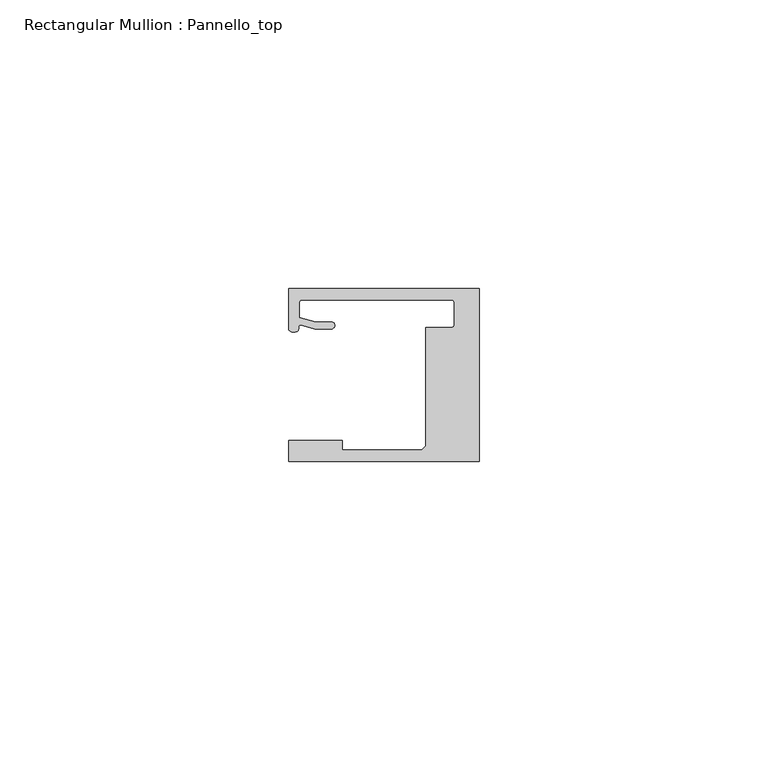
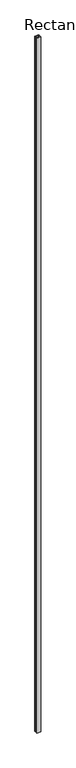
"""IFC4 building model written with IfcOpenShell, lengths in millimetres: member geometry, Rectangular Mullion : Pannello_top."""

from ifc_helpers import new_model, si_unit, frame, origin, place, context, project, spatial, polyline, circle_curve, source, transform, mapped, element, save
from ifc_brep_helpers import plane_surface, cylinder_surface, revolved_surface, extruded_surface, spline_curve, advanced_brep


def rectangular_mullion_pannello_top_acaf2075(model_context):
    return source(origin(), model_context, "Body", "AdvancedBrep", [
        advanced_brep(
        [(-33.0, -15.0, 0.0), (0.0, -15.0, 0.0), (0.0, 15.0, 0.0), (-33.0000135, 15.0, 0.0), (-33.0000135, 8.0000472, 0.0), (-30.9223017, 8.6490241, 0.0), (-28.4999305, 7.9999523, 0.0), (-25.59998, 7.9999523, 0.0), (-25.59998, 9.1999523, 0.0), (-28.3419477, 9.1999523, 0.0), (-31.19998, 9.9657591, 0.0), (-31.19998, 12.50001, 0.0), (-30.69998, 13.00001, 0.0), (-4.7999726, 13.00001, 0.0), (-4.2999726, 12.50001, 0.0), (-4.2999726, 8.7500595, 0.0), (-4.7999726, 8.2500595, 0.0), (-9.2999726, 8.2500595, 0.0), (-9.2999726, -12.2999849, 0.0), (-10.0000103, -13.0000004, 0.0), (-23.700041, -13.0000004, 0.0), (-23.700041, -11.3000004, 0.0), (-33.0, -11.3000004, 0.0), (-33.0, -15.0, -6338.7891154), (-33.0, -11.3000004, -6338.7891154), (-23.700041, -11.3000004, -6338.7891154), (-23.700041, -13.0000004, -6338.7891154), (-10.0000103, -13.0000004, -6338.7891154), (-9.2999726, -12.2999849, -6338.7891154), (-9.2999726, 8.2500595, -6338.7891154), (-4.7999726, 8.2500595, -6338.7891154), (-4.2999726, 8.7500595, -6338.7891154), (-4.2999726, 12.50001, -6338.7891154), (-4.7999726, 13.00001, -6338.7891154), (-30.69998, 13.00001, -6338.7891154), (-31.19998, 12.50001, -6338.7891154), (-31.19998, 9.9657591, -6338.7891154), (-28.3419477, 9.1999523, -6338.7891154), (-25.59998, 9.1999523, -6338.7891154), (-25.59998, 7.9999523, -6338.7891154), (-28.4999305, 7.9999523, -6338.7891154), (-30.9223017, 8.6490241, -6338.7891154), (-33.0000135, 8.0000472, -6338.7891154), (-33.0000135, 15.0, -6338.7891154), (0.0, 15.0, -6338.7891154), (0.0, -15.0, -6338.7891154)],
        [
            (0, 1),
            (1, 2),
            (2, 3),
            (3, 4),
            (4, 5, spline_curve(3, [(-33.0000135, 8.0000472, 0.0), (-33.0000135, 7.457047519, 0.0), (-32.262327879, 7.456527435, 0.0), (-31.357433266, 7.563996614, 0.0), (-31.305645054, 7.690065204, 0.0), (-31.298563602, 8.366228555, 0.0), (-31.312054066, 8.717747958, 0.0), (-30.9223017, 8.6490241, 0.0)], [4, 2, 2, 4], [0.0, 0.0027053965905959043, 0.0058611956533709, 0.007702013405570312])),
            (5, 6),
            (6, 7),
            (7, 8, circle_curve(frame((-25.59998, 8.5999523, 0.0), z_axis=(0.0, 0.0, 1.0), x_axis=(0.0, 1.0, 0.0)), 0.6)),
            (8, 9),
            (9, 10),
            (10, 11),
            (11, 12, circle_curve(frame((-30.69998, 12.50001, 0.0), z_axis=(0.0, 0.0, -1.0), x_axis=(0.0, 1.0, 0.0)), 0.5)),
            (12, 13),
            (13, 14, circle_curve(frame((-4.7999726, 12.50001, 0.0), z_axis=(0.0, 0.0, -1.0), x_axis=(1.0, 0.0, 0.0)), 0.5)),
            (14, 15),
            (15, 16, circle_curve(frame((-4.7999726, 8.7500595, 0.0), z_axis=(0.0, 0.0, -1.0), x_axis=(0.0, -1.0, 0.0)), 0.5)),
            (16, 17),
            (17, 18),
            (18, 19),
            (19, 20),
            (20, 21),
            (21, 22),
            (22, 0),
            (23, 24),
            (24, 25),
            (25, 26),
            (26, 27),
            (27, 28),
            (28, 29),
            (29, 30),
            (30, 31, circle_curve(frame((-4.7999726, 8.7500595, -6338.7891154), z_axis=(0.0, 0.0, 1.0), x_axis=(0.0, -1.0, 0.0)), 0.5)),
            (31, 32),
            (32, 33, circle_curve(frame((-4.7999726, 12.50001, -6338.7891154), z_axis=(0.0, 0.0, 1.0), x_axis=(1.0, 0.0, 0.0)), 0.5)),
            (33, 34),
            (34, 35, circle_curve(frame((-30.69998, 12.50001, -6338.7891154), z_axis=(0.0, 0.0, 1.0), x_axis=(0.0, 1.0, 0.0)), 0.5)),
            (35, 36),
            (36, 37),
            (37, 38),
            (38, 39, circle_curve(frame((-25.59998, 8.5999523, -6338.7891154), z_axis=(0.0, 0.0, -1.0), x_axis=(0.0, 1.0, 0.0)), 0.6)),
            (39, 40),
            (40, 41),
            (41, 42, spline_curve(3, [(-30.9223017, 8.6490241, -6338.7891154), (-31.312054066, 8.717747958, -6338.7891154), (-31.298563602, 8.366228555, -6338.7891154), (-31.305645054, 7.690065204, -6338.7891154), (-31.357433266, 7.563996614, -6338.7891154), (-32.262327879, 7.456527435, -6338.7891154), (-33.0000135, 7.457047519, -6338.7891154), (-33.0000135, 8.0000472, -6338.7891154)], [4, 2, 2, 4], [0.0, 0.001840817752199412, 0.004996616814974408, 0.007702013405570312])),
            (42, 43),
            (43, 44),
            (44, 45),
            (45, 23),
            (0, 23),
            (45, 1),
            (44, 2),
            (43, 3),
            (42, 4),
            (41, 5),
            (40, 6),
            (39, 7),
            (38, 8),
            (37, 9),
            (36, 10),
            (35, 11),
            (34, 12),
            (33, 13),
            (32, 14),
            (31, 15),
            (30, 16),
            (29, 17),
            (28, 18),
            (27, 19),
            (26, 20),
            (25, 21),
            (24, 22),
        ],
        [
            plane_surface(frame((0.0, -36.2491502, 0.0), z_axis=(0.0, 0.0, 1.0), x_axis=(-1.0, 0.0, 0.0))),
            plane_surface(frame((0.0, -36.2491502, -6338.7891154), z_axis=(0.0, 0.0, -1.0), x_axis=(-1.0, 0.0, 0.0))),
            plane_surface(frame((-33.0, -15.0, 0.0), z_axis=(0.0, -1.0, 0.0), x_axis=(0.0, 0.0, -1.0))),
            plane_surface(frame((0.0, -15.0, 0.0), z_axis=(1.0, 0.0, 0.0), x_axis=(0.0, 0.0, -1.0))),
            plane_surface(frame((0.0, 15.0, 0.0), z_axis=(0.0, 1.0, 0.0), x_axis=(0.0, 0.0, -1.0))),
            plane_surface(frame((-33.0000135, 15.0, 0.0), z_axis=(-1.0, 0.0, 0.0), x_axis=(0.0, 0.0, -1.0))),
            extruded_surface(spline_curve(3, [(-33.0000135, 8.0000472, -6338.7891154), (-33.0000135, 7.457047519, -6338.7891154), (-32.262327879, 7.456527435, -6338.7891154), (-31.357433266, 7.563996614, -6338.7891154), (-31.305645054, 7.690065204, -6338.7891154), (-31.298563602, 8.366228555, -6338.7891154), (-31.312054066, 8.717747958, -6338.7891154), (-30.9223017, 8.6490241, -6338.7891154)], [4, 2, 2, 4], [0.0, 0.0027053965905959043, 0.0058611956533709, 0.007702013405570312]), (0.0, 0.0, 6338.7891154), 6338.7891154),
            plane_surface(frame((-30.9223017, 8.6490241, 0.0), z_axis=(-0.25881883200192934, -0.9659258833891746, 0.0), x_axis=(0.0, 0.0, -1.0))),
            plane_surface(frame((-28.4999305, 7.9999523, 0.0), z_axis=(0.0, -1.0, 0.0), x_axis=(0.0, 0.0, -1.0))),
            cylinder_surface(frame((-25.59998, 8.5999523, 0.0), z_axis=(0.0, 0.0, 1.0), x_axis=(0.0, 1.0, 0.0)), 0.6),
            plane_surface(frame((-25.59998, 9.1999523, 0.0), z_axis=(0.0, 1.0, 0.0), x_axis=(0.0, 0.0, -1.0))),
            plane_surface(frame((-28.3419477, 9.1999523, 0.0), z_axis=(0.25881883204288636, 0.9659258833782002, 0.0), x_axis=(0.0, 0.0, -1.0))),
            plane_surface(frame((-31.19998, 9.9657591, 0.0), z_axis=(1.0, 0.0, 0.0), x_axis=(0.0, 0.0, -1.0))),
            revolved_surface(polyline([(-30.69998, 13.00001, -6338.7891154), (-30.69998, 13.00001, 0.0)]), (-30.69998, 12.50001, 0.0), (0.0, 0.0, -1.0)),
            plane_surface(frame((-30.69998, 13.00001, 0.0), z_axis=(0.0, -1.0, 0.0), x_axis=(0.0, 0.0, -1.0))),
            revolved_surface(polyline([(-4.2999726, 12.50001, -6338.7891154), (-4.2999726, 12.50001, 0.0)]), (-4.7999726, 12.50001, 0.0), (0.0, 0.0, -1.0)),
            plane_surface(frame((-4.2999726, 12.50001, 0.0), z_axis=(-1.0, 0.0, 0.0), x_axis=(0.0, 0.0, -1.0))),
            revolved_surface(polyline([(-4.7999726, 8.2500595, -6338.7891154), (-4.7999726, 8.2500595, 0.0)]), (-4.7999726, 8.7500595, 0.0), (0.0, 0.0, -1.0)),
            plane_surface(frame((-4.7999726, 8.2500595, 0.0), z_axis=(0.0, 1.0, 0.0), x_axis=(0.0, 0.0, -1.0))),
            plane_surface(frame((-9.2999726, 8.2500595, 0.0), z_axis=(-1.0, 0.0, 0.0), x_axis=(0.0, 0.0, -1.0))),
            plane_surface(frame((-9.2999726, -12.2999849, 0.0), z_axis=(-0.7070955486277984, 0.7071180135668678, 0.0), x_axis=(0.0, 0.0, -1.0))),
            plane_surface(frame((-10.0000103, -13.0000004, 0.0), z_axis=(0.0, 1.0, 0.0), x_axis=(0.0, 0.0, -1.0))),
            plane_surface(frame((-23.700041, -13.0000004, 0.0), z_axis=(1.0, 0.0, 0.0), x_axis=(0.0, 0.0, -1.0))),
            plane_surface(frame((-23.700041, -11.3000004, 0.0), z_axis=(0.0, 1.0, 0.0), x_axis=(0.0, 0.0, -1.0))),
            plane_surface(frame((-33.0, -11.3000004, 0.0), z_axis=(-1.0, 0.0, 0.0), x_axis=(0.0, 0.0, -1.0))),
        ],
        [
            (0, [[1, 2, 3, 4, 5, 6, 7, 8, 9, 10, 11, 12, 13, 14, 15, 16, 17, 18, 19, 20, 21, 22, 23]]),
            (1, [[24, 25, 26, 27, 28, 29, 30, 31, 32, 33, 34, 35, 36, 37, 38, 39, 40, 41, 42, 43, 44, 45, 46]]),
            (2, [[-1, 47, -46, 48]]),
            (3, [[-2, -48, -45, 49]]),
            (4, [[-3, -49, -44, 50]]),
            (5, [[-4, -50, -43, 51]]),
            (6, [[-5, -51, -42, 52]]),
            (7, [[-6, -52, -41, 53]]),
            (8, [[-7, -53, -40, 54]]),
            (9, [[-8, -54, -39, 55]]),
            (10, [[-9, -55, -38, 56]]),
            (11, [[-10, -56, -37, 57]]),
            (12, [[-11, -57, -36, 58]]),
            (13, [[-12, -58, -35, 59]]),
            (14, [[-13, -59, -34, 60]]),
            (15, [[-14, -60, -33, 61]]),
            (16, [[-15, -61, -32, 62]]),
            (17, [[-16, -62, -31, 63]]),
            (18, [[-17, -63, -30, 64]]),
            (19, [[-18, -64, -29, 65]]),
            (20, [[-19, -65, -28, 66]]),
            (21, [[-20, -66, -27, 67]]),
            (22, [[-21, -67, -26, 68]]),
            (23, [[-22, -68, -25, 69]]),
            (24, [[-23, -69, -24, -47]]),
        ],
    ),
    ])


if __name__ == "__main__":
    model = new_model("IFC4")
    model_context = context("Model", 3, world=origin())
    ifc_project = project(units=[si_unit("LENGTHUNIT", "METRE", prefix="MILLI")], contexts=[model_context])
    site = spatial("IfcSite", under=ifc_project)
    building = spatial("IfcBuilding", under=site)
    placement = place(None, origin())
    rectangular_mullion_pannello_top_shape = rectangular_mullion_pannello_top_acaf2075(model_context)
    element("IfcMember", 1, ObjectType="Rectangular Mullion : Pannello_top", at=placement, inside=building, context=model_context, shape_type="MappedRepresentation", body=[
        mapped(rectangular_mullion_pannello_top_shape, transform((0.0, 0.0, 0.0), x_axis=(1.0, 0.0, 0.0), y_axis=(0.0, 1.0, 0.0), z_axis=(0.0, 0.0, 1.0))),
    ])
    save(model, "model.ifc")

# Revit data of these elements
# Type "Rectangular Mullion : Pannello_top"
#   built-in parameter 1007322 = 0.0984252 (stored number, unit not read)
#   built-in parameter 1007321 = 0 (stored number, unit not read)
#   built-in parameter 1007320 = 0.0305117 (stored number, unit not read)
